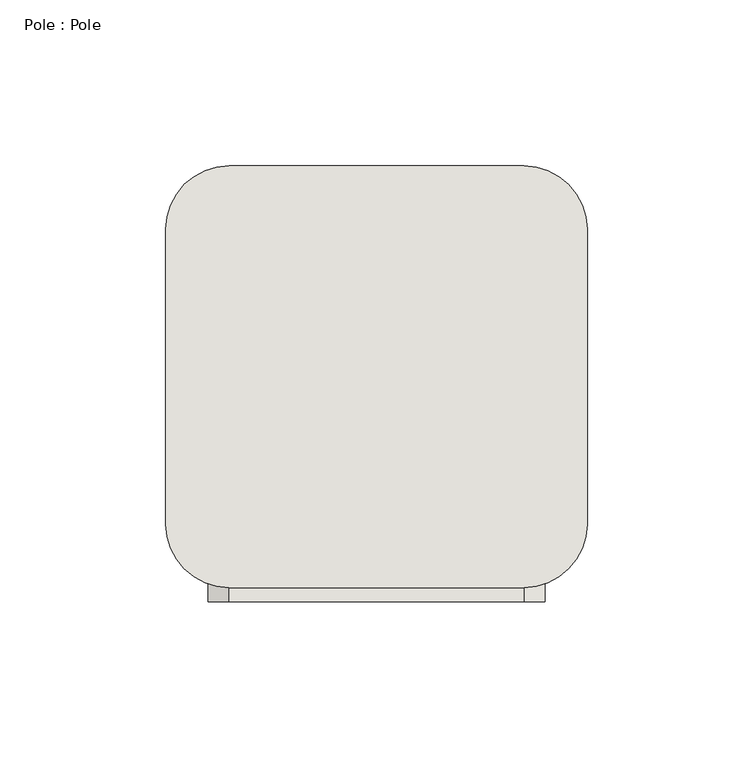
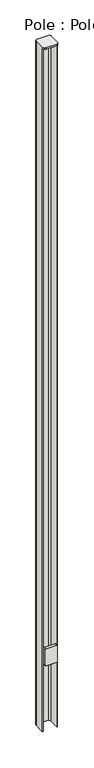
"""IFC4 building model written with IfcOpenShell, lengths in millimetres: wall geometry, Pole : Pole."""

from ifc_helpers import new_model, si_unit, point, frame, frame_2d, origin, place, context, project, spatial, polyline, circle_curve, trimmed, segment, composite_curve, outline, extrude, source, transform, mapped, element, save
from ifc_brep_helpers import plane_surface, cylinder_surface, revolved_surface, advanced_brep


def pole_pole_e244cbc8(model_context):
    return source(origin(), model_context, "Body", "SolidModel", [
        extrude(outline(composite_curve([segment(trimmed(circle_curve(frame_2d((1524.0, 40320.9125)), 6.35), [point((1530.35, 40320.9125))], [point((1524.0, 40314.5625))], False, "CARTESIAN"), True, "CONTINUOUS"), segment(polyline([(1524.0, 40314.5625), (1384.3, 40314.5625)]), True, "CONTINUOUS"), segment(trimmed(circle_curve(frame_2d((1384.3, 40320.9125)), 6.35), [point((1384.3, 40314.5625))], [point((1377.95, 40320.9125))], False, "CARTESIAN"), True, "CONTINUOUS"), segment(polyline([(1377.95, 40320.9125), (1377.95, 40409.8125)]), True, "CONTINUOUS"), segment(trimmed(circle_curve(frame_2d((1384.3, 40409.8125)), 6.35), [point((1377.95, 40409.8125))], [point((1384.3, 40416.1625))], False, "CARTESIAN"), True, "CONTINUOUS"), segment(polyline([(1384.3, 40416.1625), (1524.0, 40416.1625)]), True, "CONTINUOUS"), segment(trimmed(circle_curve(frame_2d((1524.0, 40409.8125)), 6.35), [point((1524.0, 40416.1625))], [point((1530.35, 40409.8125))], False, "CARTESIAN"), True, "CONTINUOUS"), segment(polyline([(1530.35, 40409.8125), (1530.35, 40320.9125)]), True, "CONTINUOUS")], self_intersect=False)), frame((0.0, 533.8687274, 0.0), z_axis=(0.0, 1.0, 0.0), x_axis=(0.0, 0.0, 1.0)), (0.0, 0.0, 1.0), 21.6991295),
        advanced_brep(
        [(40409.8125, 664.1825707, 787.4), (40428.8625, 645.1325707, 787.4), (40428.8625, 556.2325707, 787.4), (40422.5125, 556.2325707, 787.4), (40422.5125, 645.1325707, 787.4), (40409.8125, 657.8325707, 787.4), (40320.9125, 657.8325707, 787.4), (40308.2125, 645.1325707, 787.4), (40308.2125, 556.2325707, 787.4), (40301.8625, 556.2325707, 787.4), (40301.8625, 645.1325707, 787.4), (40320.9125, 664.1825707, 787.4), (40320.9125, 664.1825707, 6845.3), (40320.9125, 664.1825707, 6858.0), (40409.8125, 664.1825707, 6858.0), (40409.8125, 664.1825707, 6845.3), (40301.8625, 645.1325707, 6845.3), (40301.8625, 556.2325707, 6845.3), (40301.8625, 556.2325707, 6858.0), (40301.8625, 645.1325707, 6858.0), (40428.8625, 645.1325707, 6845.3), (40428.8625, 645.1325707, 6858.0), (40428.8625, 556.2325707, 6858.0), (40428.8625, 556.2325707, 6845.3), (40308.2125, 645.1325707, 6845.3), (40308.2125, 556.2325707, 6845.3), (40320.9125, 657.8325707, 6845.3), (40409.8125, 657.8325707, 6845.3), (40422.5125, 645.1325707, 6845.3), (40422.5125, 556.2325707, 6845.3), (40320.9125, 537.1825707, 6858.0), (40409.8125, 537.1825707, 6858.0), (40409.8125, 537.1825707, 6845.3), (40320.9125, 537.1825707, 6845.3)],
        [
            (0, 1, circle_curve(frame((40409.8125, 645.1325707, 787.4), z_axis=(0.0, 0.0, -1.0), x_axis=(1.0, 0.0, 0.0)), 19.05)),
            (1, 2),
            (2, 3),
            (3, 4),
            (4, 5, circle_curve(frame((40409.8125, 645.1325707, 787.4), z_axis=(0.0, 0.0, 1.0), x_axis=(1.0, 0.0, 0.0)), 12.7)),
            (5, 6),
            (6, 7, circle_curve(frame((40320.9125, 645.1325707, 787.4), z_axis=(0.0, 0.0, 1.0), x_axis=(1.0, 0.0, 0.0)), 12.7)),
            (7, 8),
            (8, 9),
            (9, 10),
            (10, 11, circle_curve(frame((40320.9125, 645.1325707, 787.4), z_axis=(0.0, 0.0, -1.0), x_axis=(1.0, 0.0, 0.0)), 19.05)),
            (11, 0),
            (11, 12),
            (12, 13),
            (13, 14),
            (14, 15),
            (15, 0),
            (10, 16),
            (16, 12, circle_curve(frame((40320.9125, 645.1325707, 6845.3), z_axis=(0.0, 0.0, -1.0), x_axis=(1.0, 0.0, 0.0)), 19.05)),
            (9, 17),
            (17, 18),
            (18, 19),
            (19, 16),
            (1, 20),
            (20, 21),
            (21, 22),
            (22, 23),
            (23, 2),
            (15, 20, circle_curve(frame((40409.8125, 645.1325707, 6845.3), z_axis=(0.0, 0.0, -1.0), x_axis=(1.0, 0.0, 0.0)), 19.05)),
            (7, 24),
            (24, 25),
            (25, 8),
            (6, 26),
            (26, 24, circle_curve(frame((40320.9125, 645.1325707, 6845.3), z_axis=(0.0, 0.0, 1.0), x_axis=(1.0, 0.0, 0.0)), 12.7)),
            (5, 27),
            (27, 26),
            (4, 28),
            (28, 27, circle_curve(frame((40409.8125, 645.1325707, 6845.3), z_axis=(0.0, 0.0, 1.0), x_axis=(1.0, 0.0, 0.0)), 12.7)),
            (3, 29),
            (29, 28),
            (13, 19, circle_curve(frame((40320.9125, 645.1325707, 6858.0), z_axis=(0.0, 0.0, 1.0), x_axis=(1.0, 0.0, 0.0)), 19.05)),
            (18, 30, circle_curve(frame((40320.9125, 556.2325707, 6858.0), z_axis=(0.0, 0.0, 1.0), x_axis=(1.0, 0.0, 0.0)), 19.05)),
            (30, 31),
            (31, 22, circle_curve(frame((40409.8125, 556.2325707, 6858.0), z_axis=(0.0, 0.0, 1.0), x_axis=(1.0, 0.0, 0.0)), 19.05)),
            (21, 14, circle_curve(frame((40409.8125, 645.1325707, 6858.0), z_axis=(0.0, 0.0, 1.0), x_axis=(1.0, 0.0, 0.0)), 19.05)),
            (23, 32, circle_curve(frame((40409.8125, 556.2325707, 6845.3), z_axis=(0.0, 0.0, -1.0), x_axis=(1.0, 0.0, 0.0)), 19.05)),
            (32, 33),
            (33, 17, circle_curve(frame((40320.9125, 556.2325707, 6845.3), z_axis=(0.0, 0.0, -1.0), x_axis=(1.0, 0.0, 0.0)), 19.05)),
            (17, 25),
            (29, 23),
            (33, 30),
            (32, 31),
        ],
        [
            plane_surface(frame((40301.8625, 664.1825707, 787.4), z_axis=(0.0, 0.0, -1.0), x_axis=(1.0, 0.0, 0.0))),
            plane_surface(frame((40409.8125, 664.1825707, 6845.3), z_axis=(0.0, 1.0, 0.0), x_axis=(0.0, 0.0, -1.0))),
            cylinder_surface(frame((40320.9125, 645.1325707, 787.4), z_axis=(0.0, 0.0, 1.0), x_axis=(1.0, 0.0, 0.0)), 19.05),
            plane_surface(frame((40301.8625, 645.1325707, 6845.3), z_axis=(-1.0, 0.0, 0.0), x_axis=(0.0, 0.0, -1.0))),
            plane_surface(frame((40428.8625, 556.2325707, 6845.3), z_axis=(1.0, 0.0, 0.0), x_axis=(0.0, 0.0, -1.0))),
            cylinder_surface(frame((40409.8125, 645.1325707, 787.4), z_axis=(0.0, 0.0, 1.0), x_axis=(1.0, 0.0, 0.0)), 19.05),
            plane_surface(frame((40308.2125, 556.2325707, 6845.3), z_axis=(1.0, 0.0, 0.0), x_axis=(0.0, 0.0, -1.0))),
            revolved_surface(polyline([(40333.612499999996, 645.1325707, 787.4), (40333.612499999996, 645.1325707, 6845.3)]), (40320.9125, 645.1325707, 787.4), (0.0, 0.0, -1.0)),
            plane_surface(frame((40320.9125, 657.8325707, 6845.3), z_axis=(0.0, -1.0, 0.0), x_axis=(0.0, 0.0, -1.0))),
            revolved_surface(polyline([(40422.5125, 645.1325707, 787.4), (40422.5125, 645.1325707, 6845.3)]), (40409.8125, 645.1325707, 787.4), (0.0, 0.0, -1.0)),
            plane_surface(frame((40422.5125, 645.1325707, 6845.3), z_axis=(-1.0, 0.0, 0.0), x_axis=(0.0, 0.0, -1.0))),
            plane_surface(frame((40301.8625, 664.1825707, 6858.0), z_axis=(0.0, 0.0, 1.0), x_axis=(-1.0, 0.0, 0.0))),
            plane_surface(frame((40301.8625, 664.1825707, 6845.3), z_axis=(0.0, 0.0, -1.0), x_axis=(1.0, 0.0, 0.0))),
            cylinder_surface(frame((40320.9125, 645.1325707, 6845.3), z_axis=(0.0, 0.0, 1.0), x_axis=(1.0, 0.0, 0.0)), 19.05),
            cylinder_surface(frame((40320.9125, 556.2325707, 6845.3), z_axis=(0.0, 0.0, 1.0), x_axis=(1.0, 0.0, 0.0)), 19.05),
            plane_surface(frame((40320.9125, 537.1825707, 6858.0), z_axis=(0.0, -1.0, 0.0), x_axis=(0.0, 0.0, -1.0))),
            cylinder_surface(frame((40409.8125, 556.2325707, 6845.3), z_axis=(0.0, 0.0, 1.0), x_axis=(1.0, 0.0, 0.0)), 19.05),
            cylinder_surface(frame((40409.8125, 645.1325707, 6845.3), z_axis=(0.0, 0.0, 1.0), x_axis=(1.0, 0.0, 0.0)), 19.05),
            plane_surface(frame((40301.8625, 556.2325707, 6845.3), z_axis=(0.0, -1.0, 0.0), x_axis=(0.0, 0.0, -1.0))),
            plane_surface(frame((40422.5125, 556.2325707, 6845.3), z_axis=(0.0, -1.0, 0.0), x_axis=(0.0, 0.0, -1.0))),
        ],
        [
            (0, [[1, 2, 3, 4, 5, 6, 7, 8, 9, 10, 11, 12]]),
            (1, [[-12, 13, 14, 15, 16, 17]]),
            (2, [[-11, 18, 19, -13]]),
            (3, [[-10, 20, 21, 22, 23, -18]]),
            (4, [[-2, 24, 25, 26, 27, 28]]),
            (5, [[-1, -17, 29, -24]]),
            (6, [[-8, 30, 31, 32]]),
            (7, [[-7, 33, 34, -30]]),
            (8, [[-6, 35, 36, -33]]),
            (9, [[-5, 37, 38, -35]]),
            (10, [[-4, 39, 40, -37]]),
            (11, [[-15, 41, -22, 42, 43, 44, -26, 45]]),
            (12, [[46, 47, 48, 49, -31, -34, -36, -38, -40, 50]]),
            (13, [[-41, -14, -19, -23]]),
            (14, [[-42, -21, -48, 51]]),
            (15, [[-43, -51, -47, 52]]),
            (16, [[-44, -52, -46, -27]]),
            (17, [[-45, -25, -29, -16]]),
            (18, [[-9, -32, -49, -20]]),
            (19, [[-3, -28, -50, -39]]),
        ],
    ),
    ])


if __name__ == "__main__":
    model = new_model("IFC4")
    model_context = context("Model", 3, world=origin())
    ifc_project = project(units=[si_unit("LENGTHUNIT", "METRE", prefix="MILLI")], contexts=[model_context])
    site = spatial("IfcSite", under=ifc_project)
    building = spatial("IfcBuilding", under=site)
    placement = place(None, origin())
    pole_pole_shape = pole_pole_e244cbc8(model_context)
    element("IfcWall", 1, ObjectType="Pole : Pole", at=placement, inside=building, context=model_context, shape_type="MappedRepresentation", body=[
        mapped(pole_pole_shape, transform((0.0, 0.0, 0.0), x_axis=(1.0, 0.0, 0.0), y_axis=(0.0, 1.0, 0.0), z_axis=(0.0, 0.0, 1.0))),
    ])
    save(model, "model.ifc")

# Revit data of these elements
# Element 1 (IfcWall, "Pole : Pole")
#   Materials on its faces: "5\" STRAIGHT SQUARE STEEL LIGHT POLE", "HANDHOLE WITH 4x6\" COVER"
# Materials
#   "5\" STRAIGHT SQUARE STEEL LIGHT POLE": class "Metal", colour RGB 199 199 199, transparency 0, Description = "Carbon steel", Cost = 0
#   "HANDHOLE WITH 4x6\" COVER": class "Metal", colour RGB 199 199 199, transparency 0, Description = "Carbon steel", Cost = 0
